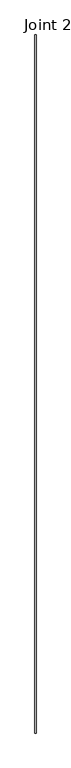
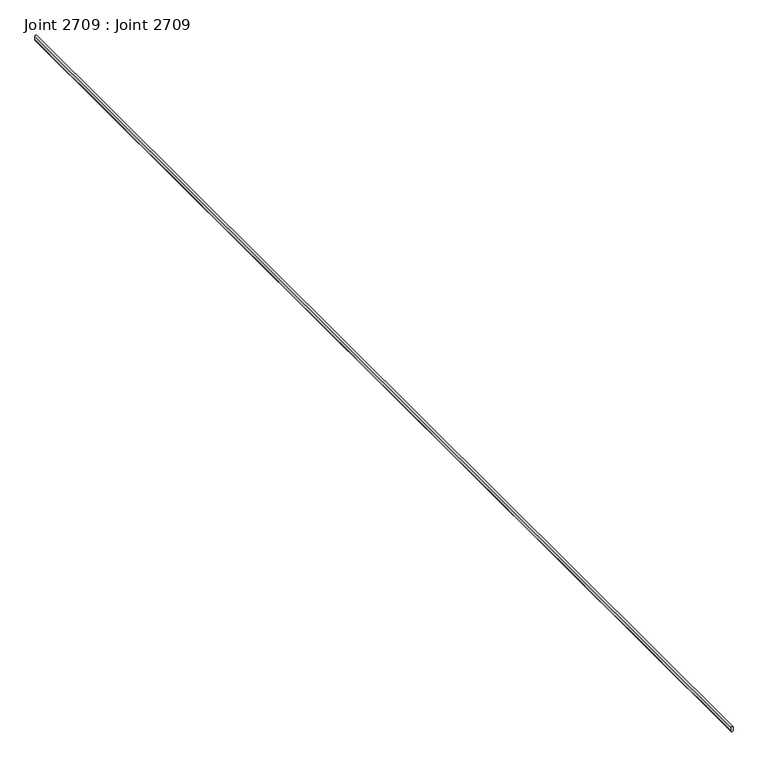
"""IFC4 building model written with IfcOpenShell, lengths in millimetres: proxy geometry, Joint 2709 : Joint 2709."""

import ifcopenshell
import ifcopenshell.guid

model = None  # the IFC model being written
_history = None  # IfcOwnerHistory: only IFC2X3 demands one
_inside = {}  # id of a spatial element -> (the spatial element, [elements in it])
_under = {}  # id of a project, library or spatial element -> (it, [spatial elements below it])
_declared = {}  # id of a project -> (the project, [libraries it declares])
_typed = {}  # id of a type object -> (the type object, [elements of that type])
_made_of = {}  # id of a material, layer set ... -> (it, [elements and type objects made of it])


def new_model(schema):
    """Start an empty IFC model of exactly this schema.

    Asked for "IFC4X3", IfcOpenShell would pick the latest addendum, in which some entities
    have other attributes; the version numbers below select the first issue.
    IFC2X3 requires an IfcOwnerHistory on every rooted entity: one is made here for all.
    """
    global model, _history
    if schema == "IFC4X3":
        model = ifcopenshell.file(schema_version=(4, 3, 0, 0))
    else:
        model = ifcopenshell.file(schema=schema)
    _inside.clear()
    _under.clear()
    _declared.clear()
    _typed.clear()
    _made_of.clear()
    _history = None
    if model.schema == "IFC2X3":
        org = make("IfcOrganization", Name="unknown")
        user = make(
            "IfcPersonAndOrganization",
            ThePerson=make("IfcPerson", FamilyName="unknown"),
            TheOrganization=org,
        )
        app = make(
            "IfcApplication",
            ApplicationDeveloper=org,
            Version="unknown",
            ApplicationFullName="unknown",
            ApplicationIdentifier="unknown",
        )
        _history = make(
            "IfcOwnerHistory",
            OwningUser=user,
            OwningApplication=app,
            ChangeAction="ADDED",
            CreationDate=0,
        )
    return model


def make(cls, **values):
    """One entity of the class cls with the attributes given. An attribute that is None is left unset."""
    return model.create_entity(
        cls, **{name: value for name, value in values.items() if value is not None}
    )


def rooted(cls, **values):
    """An entity with a GlobalId (a new one), such as an element, a storey or a relation."""
    return make(cls, GlobalId=ifcopenshell.guid.new(), OwnerHistory=_history, **values)


def si_unit(unit_type, name, prefix=None):
    """IfcSIUnit, for example si_unit("LENGTHUNIT", "METRE", prefix="MILLI")."""
    return make("IfcSIUnit", UnitType=unit_type, Prefix=prefix, Name=name)


def assignment(units):
    """IfcUnitAssignment: the units of a project."""
    return None if units is None else make("IfcUnitAssignment", Units=units)


def point(xyz):
    """IfcCartesianPoint."""
    return None if xyz is None else make("IfcCartesianPoint", Coordinates=xyz)


def direction(xyz):
    """IfcDirection."""
    return None if xyz is None else make("IfcDirection", DirectionRatios=xyz)


def frame(location, z_axis=None, x_axis=None):
    """IfcAxis2Placement3D, a coordinate frame: its origin and axes. An axis left out is left unset."""
    return make(
        "IfcAxis2Placement3D",
        Location=point(location),
        Axis=direction(z_axis),
        RefDirection=direction(x_axis),
    )


def frame_2d(location, x_axis=None):
    """IfcAxis2Placement2D, a coordinate frame in the plane: its origin and x axis."""
    return make(
        "IfcAxis2Placement2D", Location=point(location), RefDirection=direction(x_axis)
    )


def origin():
    """The frame at (0, 0, 0) with its axes left unset."""
    return frame((0.0, 0.0, 0.0))


def place(relative_to, where):
    """IfcLocalPlacement: puts the frame where relative to a parent placement (None: the world)."""
    return make(
        "IfcLocalPlacement", PlacementRelTo=relative_to, RelativePlacement=where
    )


def context(
    kind, dimensions, precision=None, world=None, true_north=None, identifier=None
):
    """IfcGeometricRepresentationContext, for example the 3D "Model" context."""
    return make(
        "IfcGeometricRepresentationContext",
        ContextIdentifier=identifier,
        ContextType=kind,
        CoordinateSpaceDimension=dimensions,
        Precision=precision,
        WorldCoordinateSystem=world,
        TrueNorth=true_north,
    )


def project(units=None, contexts=None):
    """IfcProject with its units and contexts."""
    return rooted(
        "IfcProject",
        Name="project",
        RepresentationContexts=contexts,
        UnitsInContext=assignment(units),
    )


def spatial(cls, under=None, at=None, **own):
    """A site, building, storey or space (cls), placed at a placement, below another one or the project."""
    s = rooted(cls, ObjectPlacement=at, **own)
    if under is not None:
        _under.setdefault(under.id(), (under, []))[1].append(s)
    return s


def polyline(points):
    """IfcPolyline through the points."""
    return make("IfcPolyline", Points=[point(p) for p in points])


def circle_curve(where, radius):
    """IfcCircle in the frame where."""
    return make("IfcCircle", Position=where, Radius=radius)


def trimmed(basis, trim1, trim2, sense, master):
    """IfcTrimmedCurve: the piece of a basis curve between two trims."""
    return make(
        "IfcTrimmedCurve",
        BasisCurve=basis,
        Trim1=trim1,
        Trim2=trim2,
        SenseAgreement=sense,
        MasterRepresentation=master,
    )


def segment(curve, same_sense, transition):
    """IfcCompositeCurveSegment."""
    return make(
        "IfcCompositeCurveSegment",
        Transition=transition,
        SameSense=same_sense,
        ParentCurve=curve,
    )


def composite_curve(segments, self_intersect=None):
    """IfcCompositeCurve: segments joined end to end."""
    return make("IfcCompositeCurve", Segments=segments, SelfIntersect=self_intersect)


def outline(outer, holes=None, kind="AREA"):
    """IfcArbitraryClosedProfileDef: a profile drawn as a closed curve; with holes, ...WithVoids."""
    if holes is None:
        return make("IfcArbitraryClosedProfileDef", ProfileType=kind, OuterCurve=outer)
    return make(
        "IfcArbitraryProfileDefWithVoids",
        ProfileType=kind,
        OuterCurve=outer,
        InnerCurves=holes,
    )


def extrude(swept, where, along, depth):
    """IfcExtrudedAreaSolid: the profile swept, set in the frame where, extruded along a direction by depth."""
    return make(
        "IfcExtrudedAreaSolid",
        SweptArea=swept,
        Position=where,
        ExtrudedDirection=direction(along),
        Depth=depth,
    )


def shape(context_of_items, identifier, shape_type, items):
    """IfcShapeRepresentation: the items that make up one representation, for example the "Body"."""
    return make(
        "IfcShapeRepresentation",
        ContextOfItems=context_of_items,
        RepresentationIdentifier=identifier,
        RepresentationType=shape_type,
        Items=items,
    )


def source(mapping_origin, context_of_items, identifier, shape_type, items):
    """IfcRepresentationMap: a shape defined once, which mapped items show again and again."""
    return make(
        "IfcRepresentationMap",
        MappingOrigin=mapping_origin,
        MappedRepresentation=shape(context_of_items, identifier, shape_type, items),
    )


def transform(
    local_origin,
    x_axis=None,
    y_axis=None,
    z_axis=None,
    scale=None,
    scale2=None,
    scale3=None,
    uniform=True,
):
    """IfcCartesianTransformationOperator3D, or its non-uniform kind. x_axis, y_axis, z_axis: its Axis1, 2, 3."""
    if uniform:
        return make(
            "IfcCartesianTransformationOperator3D",
            Axis1=direction(x_axis),
            Axis2=direction(y_axis),
            LocalOrigin=point(local_origin),
            Scale=scale,
            Axis3=direction(z_axis),
        )
    return make(
        "IfcCartesianTransformationOperator3DnonUniform",
        Axis1=direction(x_axis),
        Axis2=direction(y_axis),
        LocalOrigin=point(local_origin),
        Scale=scale,
        Axis3=direction(z_axis),
        Scale2=scale2,
        Scale3=scale3,
    )


def mapped(mapping_source, mapping_target):
    """IfcMappedItem: shows the shape of a source again, moved by a transform."""
    return make(
        "IfcMappedItem", MappingSource=mapping_source, MappingTarget=mapping_target
    )


def made_of(thing, what):
    """Note that an element or type object is made of a material, layer set ...; save() writes the relation."""
    if what is not None:
        _made_of.setdefault(what.id(), (what, []))[1].append(thing)
    return thing


def element(
    cls,
    number,
    at=None,
    inside=None,
    cuts=None,
    type_object=None,
    material=None,
    context=None,
    identifier="Body",
    shape_type=None,
    held_by="IfcProductDefinitionShape",
    body=None,
    shapes=None,
    **own,
):
    """One element of the class cls, such as IfcWall. Its Tag is "e" and its number.

    at: its placement. inside: the storey or other place that contains it. cuts: it is an
    opening in that element (IfcRelVoidsElement). A single representation is given by context,
    identifier, shape_type and body (its items); several are given by shapes. held_by: the class
    of the entity that holds the representations. save() writes the other relations.
    """
    e = rooted(cls, Tag="e%d" % number, ObjectPlacement=at, **own)
    if body is not None:
        shapes = [shape(context, identifier, shape_type, body)]
    if shapes is not None:
        e.Representation = make(held_by, Representations=shapes)
    if inside is not None:
        _inside.setdefault(inside.id(), (inside, []))[1].append(e)
    if cuts is not None:
        rooted(
            "IfcRelVoidsElement", RelatingBuildingElement=cuts, RelatedOpeningElement=e
        )
    if type_object is not None:
        _typed.setdefault(type_object.id(), (type_object, []))[1].append(e)
    return made_of(e, material)


def aggregate(whole, parts):
    """IfcRelAggregates: a whole, such as a stair, and the parts it consists of."""
    return rooted("IfcRelAggregates", RelatingObject=whole, RelatedObjects=parts)


def save(model, path):
    """Write the relations noted so far, then the file.

    IfcRelAggregates (storeys below a building ...), IfcRelContainedInSpatialStructure (elements
    in a storey), IfcRelDefinesByType, IfcRelAssociatesMaterial and IfcRelDeclares: one each for
    every whole, place, type object, material and project.
    """
    for whole, parts in _under.values():
        aggregate(whole, parts)
    for where, things in _inside.values():
        rooted(
            "IfcRelContainedInSpatialStructure",
            RelatedElements=things,
            RelatingStructure=where,
        )
    for kind, things in _typed.values():
        rooted("IfcRelDefinesByType", RelatedObjects=things, RelatingType=kind)
    for what, things in _made_of.values():
        rooted("IfcRelAssociatesMaterial", RelatedObjects=things, RelatingMaterial=what)
    for by, libraries in _declared.values():
        rooted("IfcRelDeclares", RelatingContext=by, RelatedDefinitions=libraries)
    model.write(path)


def joint_2709_joint_2709_9d0f0c8f(model_context):
    return source(origin(), model_context, "Body", "SweptSolid", [
        extrude(outline(composite_curve([segment(polyline([(40328.7531984, -1061.7883298), (40334.7081544, -1061.7883298)]), True, "CONTINUOUS"), segment(trimmed(circle_curve(frame_2d((40334.7081544, -1063.3742673)), 1.5859375), [point((40334.7081544, -1061.7883298))], [point((40334.7081544, -1064.9602048))], False, "CARTESIAN"), True, "CONTINUOUS"), segment(polyline([(40334.7081544, -1064.9602048), (40328.7531984, -1064.9602048)]), True, "CONTINUOUS"), segment(trimmed(circle_curve(frame_2d((40328.7531984, -1063.3742673)), 1.5859375), [point((40328.7531984, -1064.9602048))], [point((40328.7531984, -1061.7883298))], False, "CARTESIAN"), True, "CONTINUOUS")], self_intersect=False)), frame((0.0, -1052.8906574, 0.0), z_axis=(0.0, 1.0, 0.0), x_axis=(0.0, 0.0, 1.0)), (0.0, 0.0, 1.0), 2000.0),
    ])


if __name__ == "__main__":
    model = new_model("IFC4")
    model_context = context("Model", 3, world=origin())
    ifc_project = project(units=[si_unit("LENGTHUNIT", "METRE", prefix="MILLI")], contexts=[model_context])
    site = spatial("IfcSite", under=ifc_project)
    building = spatial("IfcBuilding", under=site)
    placement = place(None, origin())
    joint_2709_joint_2709_shape = joint_2709_joint_2709_9d0f0c8f(model_context)
    element("IfcBuildingElementProxy", 1, Name="Joint 2709 : Joint 2709", ObjectType="Joint 2709 : Joint 2709", at=placement, inside=building, context=model_context, shape_type="MappedRepresentation", body=[
        mapped(joint_2709_joint_2709_shape, transform((0.0, 0.0, 0.0), x_axis=(1.0, 0.0, 0.0), y_axis=(0.0, 1.0, 0.0), z_axis=(0.0, 0.0, 1.0))),
    ])
    save(model, "model.ifc")

# Revit data of these elements
# Type "Joint 2709 : Joint 2709"
#   NameOverride = "Joint"
# Element 1 (IfcBuildingElementProxy, "Joint 2709 : Joint 2709")
#   Materials on its faces: "SILICON JOINT"
# Materials
#   "SILICON JOINT": class "Unassigned", colour RGB 150 184 127, transparency 0
